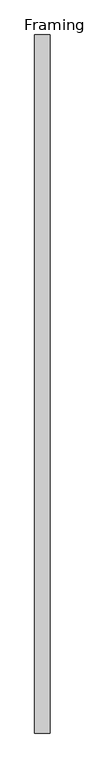
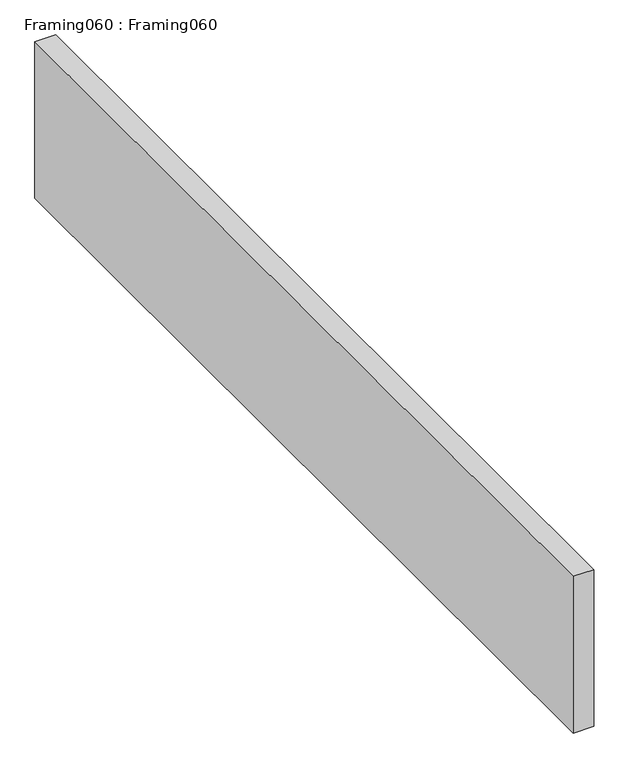
"""IFC4 building model written with IfcOpenShell, lengths in millimetres: proxy geometry, Framing060 : Framing060."""

from ifc_helpers import new_model, si_unit, frame, origin, place, context, project, spatial, polyline, outline, extrude, source, transform, mapped, element, save


def framing060_framing060_139d58be(model_context):
    return source(origin(), model_context, "Body", "SweptSolid", [
        extrude(outline(polyline([(-1793.3519086, -1052.8906574), (-1837.8019086, -1052.8906574), (-1837.8019086, 947.1093426), (-1793.3519086, 947.1093426), (-1793.3519086, -1052.8906574)])), frame((0.0, 0.0, 42133.8036692), z_axis=(0.0, 0.0, 1.0), x_axis=(1.0, 0.0, 0.0)), (0.0, 0.0, 1.0), 355.2981173),
    ])


if __name__ == "__main__":
    model = new_model("IFC4")
    model_context = context("Model", 3, world=origin())
    ifc_project = project(units=[si_unit("LENGTHUNIT", "METRE", prefix="MILLI")], contexts=[model_context])
    site = spatial("IfcSite", under=ifc_project)
    building = spatial("IfcBuilding", under=site)
    placement = place(None, origin())
    framing060_framing060_shape = framing060_framing060_139d58be(model_context)
    element("IfcBuildingElementProxy", 1, Name="Framing060 : Framing060", ObjectType="Framing060 : Framing060", at=placement, inside=building, context=model_context, shape_type="MappedRepresentation", body=[
        mapped(framing060_framing060_shape, transform((0.0, 0.0, 0.0), x_axis=(1.0, 0.0, 0.0), y_axis=(0.0, 1.0, 0.0), z_axis=(0.0, 0.0, 1.0))),
    ])
    save(model, "model.ifc")

# Revit data of these elements
# Type "Framing060 : Framing060"
#   NameOverride = "Framing060"
# Element 1 (IfcBuildingElementProxy, "Framing060 : Framing060")
#   Materials on its faces: "WOOD FRAMING (SEE STRUCT DWGS)"
# Materials
#   "WOOD FRAMING (SEE STRUCT DWGS)": class "Unassigned", colour RGB 224 188 168, transparency 0, Cost = 0
